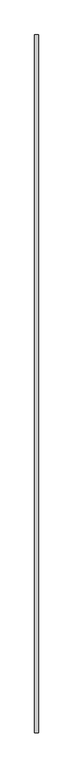
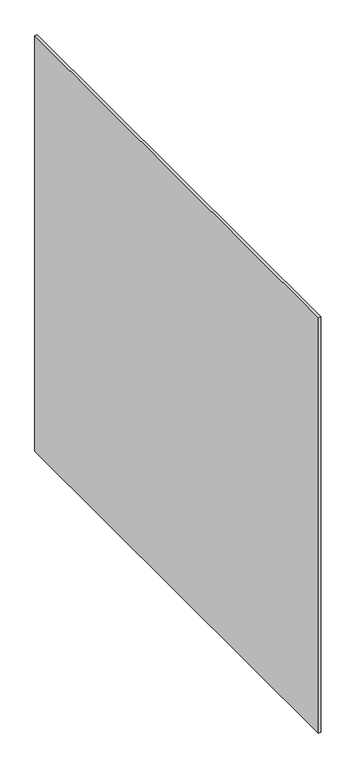
"""IFC4 building model written with IfcOpenShell, lengths in millimetres: proxy geometry, Inner panel:Inner panel:1:Inner panel:1 : Inner panel:Inner panel:300324:300043:Inner panel:1:Inner panel:1 : Inner panel:Inner panel:300324:300043 : Inner panel:Inner panel:1:Inner panel:1 : Inner panel:Inner panel:300324:300043:33 : Inner panel:Inner panel:1:Inner panel:1 : Inner panel:Inner panel:300324:300043:Inner panel:1:Inner panel:1 : Inner panel:Inner panel:300324:300043 : Inner panel:Inner panel:1:Inner panel:1 : Inner panel:Inner panel:300324:300043:300031."""

from ifc_helpers import new_model, si_unit, frame, origin, place, context, project, spatial, polyline, outline, extrude, source, transform, mapped, element, save


def generic_models_70401630(model_context):
    return source(origin(), model_context, "Body", "SweptSolid", [
        extrude(outline(polyline([(579307.711724, -576279.7163841), (579320.4117239, -576279.7163841), (579320.4117239, -578718.1163841), (579307.711724, -578718.1163841), (579307.711724, -576279.7163841)])), frame((0.0, 0.0, 3987.8117204), z_axis=(0.0, 0.0, 1.0), x_axis=(1.0, 0.0, 0.0)), (0.0, 0.0, 1.0), 2178.0382796),
    ])


if __name__ == "__main__":
    model = new_model("IFC4")
    model_context = context("Model", 3, world=origin())
    ifc_project = project(units=[si_unit("LENGTHUNIT", "METRE", prefix="MILLI")], contexts=[model_context])
    site = spatial("IfcSite", under=ifc_project)
    building = spatial("IfcBuilding", under=site)
    placement = place(None, origin())
    generic_models_shape = generic_models_70401630(model_context)
    element("IfcBuildingElementProxy", 1, Name="Inner panel:Inner panel:1:Inner panel:1 : Inner panel:Inner panel:300324:300043:Inner panel:1:Inner panel:1 : Inner panel:Inner panel:300324:300043 : Inner panel:Inner panel:1:Inner panel:1 : Inner panel:Inner panel:300324:300043:33 : Inner panel:Inner panel:1:Inner panel:1 : Inner panel:Inner panel:300324:300043:Inner panel:1:Inner panel:1 : Inner panel:Inner panel:300324:300043 : Inner panel:Inner panel:1:Inner panel:1 : Inner panel:Inner panel:300324:300043:300031", ObjectType="Inner panel:Inner panel:1:Inner panel:1 : Inner panel:Inner panel:300324:300043:Inner panel:1:Inner panel:1 : Inner panel:Inner panel:300324:300043 : Inner panel:Inner panel:1:Inner panel:1 : Inner panel:Inner panel:300324:300043:33 : Inner panel:Inner panel:1:Inner panel:1 : Inner panel:Inner panel:300324:300043:Inner panel:1:Inner panel:1 : Inner panel:Inner panel:300324:300043 : Inner panel:Inner panel:1:Inner panel:1 : Inner panel:Inner panel:300324:300043:300031", at=placement, inside=building, context=model_context, shape_type="MappedRepresentation", body=[
        mapped(generic_models_shape, transform((0.0, 0.0, 0.0), x_axis=(1.0, 0.0, 0.0), y_axis=(0.0, 1.0, 0.0), z_axis=(0.0, 0.0, 1.0))),
    ])
    save(model, "model.ifc")

# Revit data of these elements
# Type "Inner panel:Inner panel:1:Inner panel:1 : Inner panel:Inner panel:300324:300043:Inner panel:1:Inner panel:1 : Inner panel:Inner panel:300324:300043 : Inner panel:Inner panel:1:Inner panel:1 : Inner panel:Inner panel:300324:300043:33 : Inner panel:Inner panel:1:Inner panel:1 : Inner panel:Inner panel:300324:300043:Inner panel:1:Inner panel:1 : Inner panel:Inner panel:300324:300043 : Inner panel:Inner panel:1:Inner panel:1 : Inner panel:Inner panel:300324:300043:300031"
#   NameOverride = "Inner panel:Inner panel:1:Inner panel:1 : Inner panel:Inner panel:300324:300043:Inner panel:1:Inner panel:1 : Inner panel:Inner panel:300324:300043 : Inner panel:Inner panel:1:Inner panel:1 : Inner panel:Inner panel:300324:300043:300031"
#   ObjectTypeOverride = "Inner panel:1:Inner panel:1 : Inner panel:Inner panel:300324:300043 : Inner panel:Inner panel:1:Inner panel:1 : Inner panel:Inner panel:300324:300043"
#   Reference = "Inner panel"
#   Tag = "300031"
# Element 1 (IfcBuildingElementProxy, "Inner panel:Inner panel:1:Inner panel:1 : Inner panel:Inner panel:300324:300043:Inner panel:1:Inner panel:1 : Inner panel:Inner panel:300324:300043 : Inner panel:Inner panel:1:Inner panel:1 : Inner panel:Inner panel:300324:300043:33 : Inner panel:Inner panel:1:Inner panel:1 : Inner panel:Inner panel:300324:300043:Inner panel:1:Inner panel:1 : Inner panel:Inner panel:300324:300043 : Inner panel:Inner panel:1:Inner panel:1 : Inner panel:Inner panel:300324:300043:300031")
#   Materials on its faces: "1/2\" FIBERGLASS MAT GYPSUM PANELS"
# Materials
#   "1/2\" FIBERGLASS MAT GYPSUM PANELS": class "Generic", colour RGB 171 170 168, transparency 0, Description = "Gypsum Wall Board", Cost = 0
